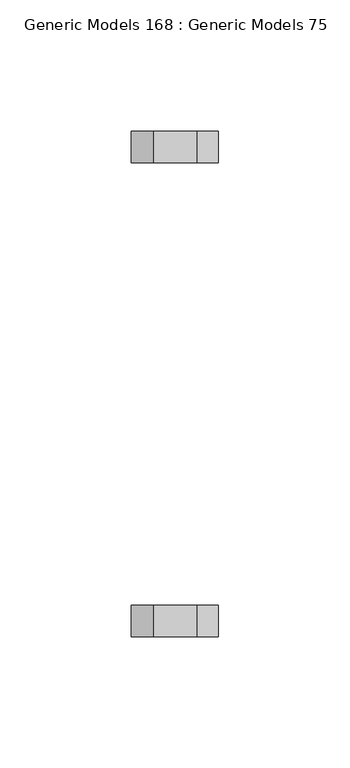
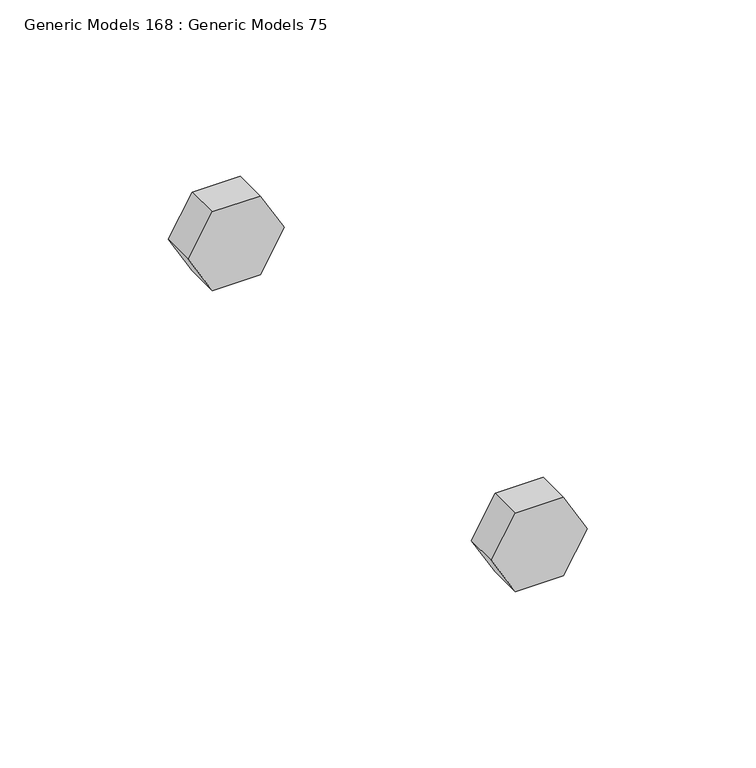
"""IFC4 building model written with IfcOpenShell, lengths in millimetres: proxy geometry, Generic Models 168 : Generic Models 75."""

from ifc_helpers import new_model, si_unit, frame, origin, place, context, project, spatial, polyline, outline, extrude, source, transform, mapped, element, save


def generic_models_168_generic_models_75_28256fc9(model_context):
    return source(origin(), model_context, "Body", "SweptSolid", [
        extrude(outline(polyline([(271505.3625, 31978.2851858), (271505.3625, 31994.7829698), (271519.65, 32003.0318618), (271533.9375, 31994.7829698), (271533.9375, 31978.2851858), (271519.65, 31970.0362939), (271505.3625, 31978.2851858)])), frame((0.0, 35193.7770442, 0.0), z_axis=(0.0, 1.0, 0.0), x_axis=(0.0, 0.0, 1.0)), (0.0, 0.0, 1.0), 11.90625),
        extrude(outline(polyline([(271505.3625, 31978.2851858), (271505.3625, 31994.7829698), (271519.65, 32003.0318618), (271533.9375, 31994.7829698), (271533.9375, 31978.2851858), (271519.65, 31970.0362939), (271505.3625, 31978.2851858)])), frame((0.0, 35373.9582942, 0.0), z_axis=(0.0, 1.0, 0.0), x_axis=(0.0, 0.0, 1.0)), (0.0, 0.0, 1.0), 11.90625),
    ])


if __name__ == "__main__":
    model = new_model("IFC4")
    model_context = context("Model", 3, world=origin())
    ifc_project = project(units=[si_unit("LENGTHUNIT", "METRE", prefix="MILLI")], contexts=[model_context])
    site = spatial("IfcSite", under=ifc_project)
    building = spatial("IfcBuilding", under=site)
    placement = place(None, origin())
    generic_models_168_generic_models_75_shape = generic_models_168_generic_models_75_28256fc9(model_context)
    element("IfcBuildingElementProxy", 1, Name="Generic Models 168 : Generic Models 75", ObjectType="Generic Models 168 : Generic Models 75", at=placement, inside=building, context=model_context, shape_type="MappedRepresentation", body=[
        mapped(generic_models_168_generic_models_75_shape, transform((0.0, 0.0, 0.0), x_axis=(1.0, 0.0, 0.0), y_axis=(0.0, 1.0, 0.0), z_axis=(0.0, 0.0, 1.0))),
    ])
    save(model, "model.ifc")

# Revit data of these elements
# Element 1 (IfcBuildingElementProxy, "Generic Models 168 : Generic Models 75")
#   Materials on its faces: "3/4\" GALV. THRU BOLTS"
# Materials
#   "3/4\" GALV. THRU BOLTS": class "Generic", colour RGB 105 69 171, transparency 0, Cost = 0
